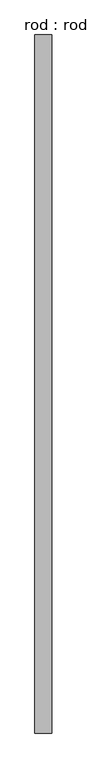
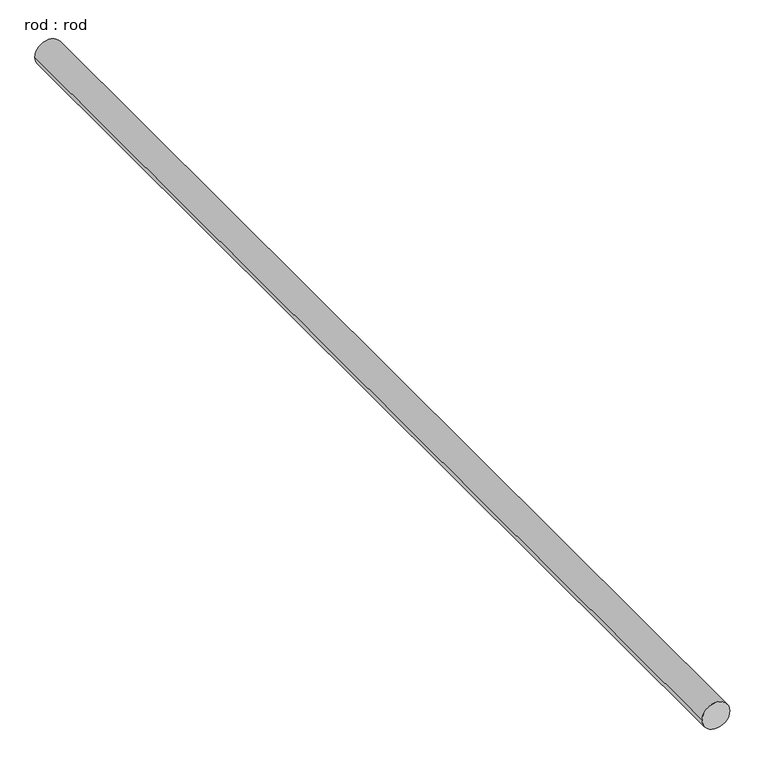
"""IFC4 building model written with IfcOpenShell, lengths in millimetres: proxy geometry, rod : rod."""

from ifc_helpers import new_model, si_unit, point, frame, frame_2d, origin, place, context, project, spatial, circle_curve, trimmed, segment, composite_curve, outline, extrude, source, transform, mapped, element, save


def rod_rod_a851ec8b(model_context):
    return source(origin(), model_context, "Body", "SweptSolid", [
        extrude(outline(composite_curve([segment(trimmed(circle_curve(frame_2d((0.0108462, 0.0)), 200.0), [point((0.0108462, 200.0))], [point((0.0108462, -200.0))], False, "CARTESIAN"), True, "CONTINUOUS"), segment(trimmed(circle_curve(frame_2d((0.0108462, 0.0)), 200.0), [point((0.0108462, -200.0))], [point((0.0108462, 200.0))], False, "CARTESIAN"), True, "CONTINUOUS")], self_intersect=False)), frame((0.0, -4268.3824958, 0.0), z_axis=(0.0, 1.0, 0.0), x_axis=(0.0, 0.0, 1.0)), (0.0, 0.0, 1.0), 16722.2222222),
    ])


if __name__ == "__main__":
    model = new_model("IFC4")
    model_context = context("Model", 3, world=origin())
    ifc_project = project(units=[si_unit("LENGTHUNIT", "METRE", prefix="MILLI")], contexts=[model_context])
    site = spatial("IfcSite", under=ifc_project)
    building = spatial("IfcBuilding", under=site)
    placement = place(None, origin())
    rod_rod_shape = rod_rod_a851ec8b(model_context)
    element("IfcBuildingElementProxy", 1, Name="rod : rod", ObjectType="rod : rod", at=placement, inside=building, context=model_context, shape_type="MappedRepresentation", body=[
        mapped(rod_rod_shape, transform((0.0, 0.0, 0.0), x_axis=(1.0, 0.0, 0.0), y_axis=(0.0, 1.0, 0.0), z_axis=(0.0, 0.0, 1.0))),
    ])
    save(model, "model.ifc")

# Revit data of these elements
# Type "rod : rod"
#   Default Elevation = 0
